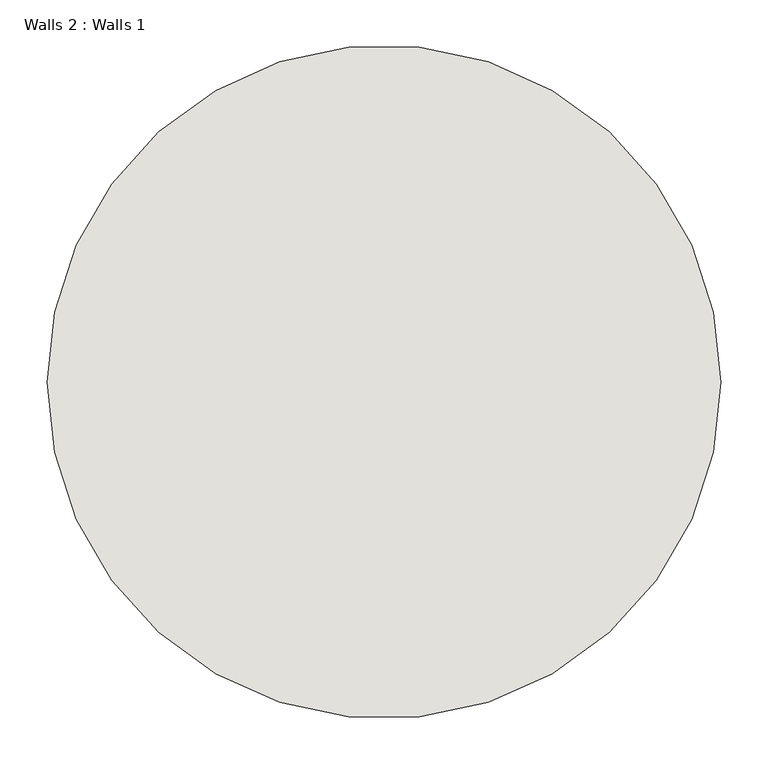
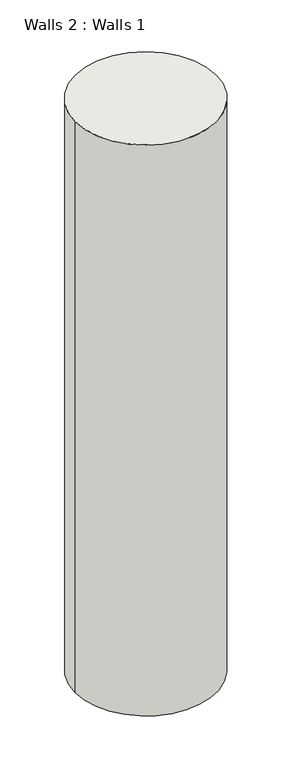
"""IFC4 building model written with IfcOpenShell, lengths in millimetres: wall geometry, Walls 2 : Walls 1."""

from ifc_helpers import new_model, si_unit, point, frame_2d, origin, origin_with_axes, place, context, project, spatial, circle_curve, trimmed, segment, composite_curve, outline, extrude, source, transform, mapped, element, save


def walls_2_walls_1_b6aa7c28(model_context):
    return source(origin(), model_context, "Body", "SweptSolid", [
        extrude(outline(composite_curve([segment(trimmed(circle_curve(frame_2d((49720.5, 33362.0236192)), 355.6), [point((49364.9, 33362.0236192))], [point((50076.1, 33362.0236192))], False, "CARTESIAN"), True, "CONTINUOUS"), segment(trimmed(circle_curve(frame_2d((49720.5, 33362.0236192)), 355.6), [point((50076.1, 33362.0236192))], [point((49364.9, 33362.0236192))], False, "CARTESIAN"), True, "CONTINUOUS")], self_intersect=False)), origin_with_axes(), (0.0, 0.0, 1.0), 3048.0),
    ])


if __name__ == "__main__":
    model = new_model("IFC4")
    model_context = context("Model", 3, world=origin())
    ifc_project = project(units=[si_unit("LENGTHUNIT", "METRE", prefix="MILLI")], contexts=[model_context])
    site = spatial("IfcSite", under=ifc_project)
    building = spatial("IfcBuilding", under=site)
    placement = place(None, origin())
    walls_2_walls_1_shape = walls_2_walls_1_b6aa7c28(model_context)
    element("IfcWall", 1, ObjectType="Walls 2 : Walls 1", at=placement, inside=building, context=model_context, shape_type="MappedRepresentation", body=[
        mapped(walls_2_walls_1_shape, transform((0.0, 0.0, 0.0), x_axis=(1.0, 0.0, 0.0), y_axis=(0.0, 1.0, 0.0), z_axis=(0.0, 0.0, 1.0))),
    ])
    save(model, "model.ifc")

# Revit data of these elements
# Element 1 (IfcWall, "Walls 2 : Walls 1")
#   Materials on its faces: "Default Wall"
# Materials
#   "Default Wall": class "Miscellaneous", colour RGB 255 255 255, transparency 0, Cost = 0
